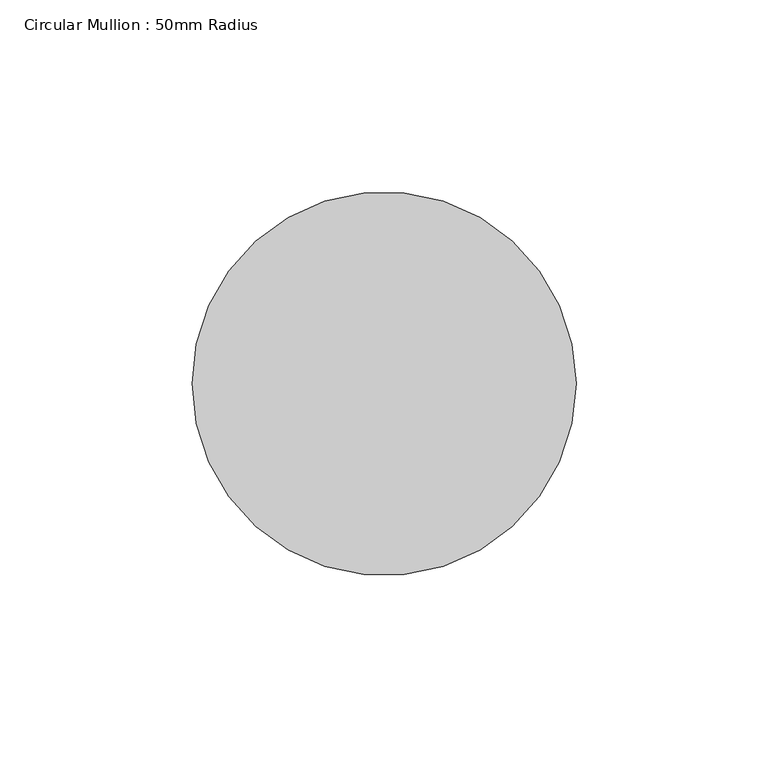
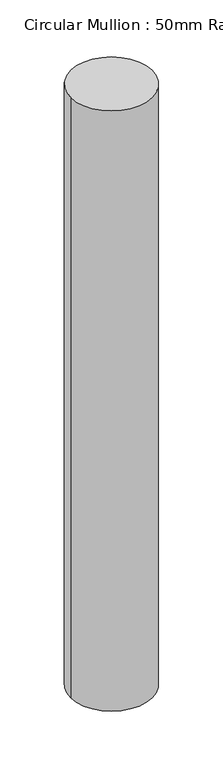
"""IFC4 building model written with IfcOpenShell, lengths in millimetres: member geometry, Circular Mullion : 50mm Radius."""

from ifc_helpers import new_model, si_unit, point, frame, frame_2d, origin, place, context, project, spatial, circle_curve, trimmed, segment, composite_curve, outline, extrude, source, transform, mapped, element, save


def circular_mullion_50mm_radius_ce80b61f(model_context):
    return source(origin(), model_context, "Body", "SweptSolid", [
        extrude(outline(composite_curve([segment(trimmed(circle_curve(frame_2d((-50.0, 0.0)), 50.0), [point((0.0, 0.0))], [point((-100.0, 0.0))], False, "CARTESIAN"), True, "CONTINUOUS"), segment(trimmed(circle_curve(frame_2d((-50.0, 0.0)), 50.0), [point((-100.0, 0.0))], [point((0.0, 0.0))], False, "CARTESIAN"), True, "CONTINUOUS")], self_intersect=False)), frame((0.0, 0.0, -778.4939902), z_axis=(0.0, 0.0, 1.0), x_axis=(1.0, 0.0, 0.0)), (0.0, 0.0, 1.0), 778.4939902),
    ])


if __name__ == "__main__":
    model = new_model("IFC4")
    model_context = context("Model", 3, world=origin())
    ifc_project = project(units=[si_unit("LENGTHUNIT", "METRE", prefix="MILLI")], contexts=[model_context])
    site = spatial("IfcSite", under=ifc_project)
    building = spatial("IfcBuilding", under=site)
    placement = place(None, origin())
    circular_mullion_50mm_radius_shape = circular_mullion_50mm_radius_ce80b61f(model_context)
    element("IfcMember", 1, ObjectType="Circular Mullion : 50mm Radius", at=placement, inside=building, context=model_context, shape_type="MappedRepresentation", body=[
        mapped(circular_mullion_50mm_radius_shape, transform((0.0, 0.0, 0.0), x_axis=(1.0, 0.0, 0.0), y_axis=(0.0, 1.0, 0.0), z_axis=(0.0, 0.0, 1.0))),
    ])
    save(model, "model.ifc")

# Revit data of these elements
# Type "Circular Mullion : 50mm Radius"
#   built-in parameter 1007350 = 0.164042 (stored number, unit not read)
# Element 1 (IfcMember, "Circular Mullion : 50mm Radius")
#   Materials on its faces: "Aluminium"
# Materials
#   "Aluminium": class "Metal", colour RGB 247 247 247, transparency 0, Description = "Aluminium 6061", Cost = 0
